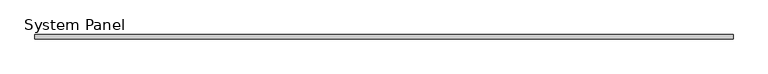
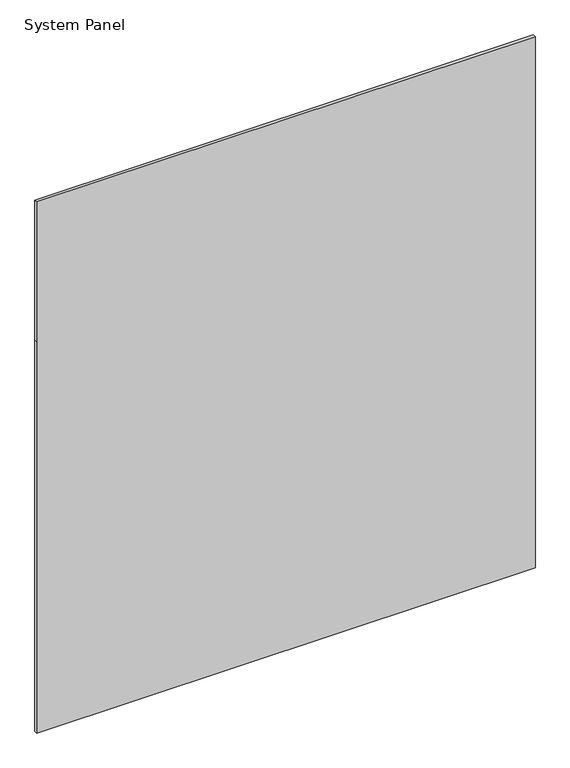
"""IFC4 building model written with IfcOpenShell, lengths in millimetres: plate geometry, System Panel : 로이복층유리_16."""

import ifcopenshell
import ifcopenshell.guid

model = None  # the IFC model being written
_history = None  # IfcOwnerHistory: only IFC2X3 demands one
_inside = {}  # id of a spatial element -> (the spatial element, [elements in it])
_under = {}  # id of a project, library or spatial element -> (it, [spatial elements below it])
_declared = {}  # id of a project -> (the project, [libraries it declares])
_typed = {}  # id of a type object -> (the type object, [elements of that type])
_made_of = {}  # id of a material, layer set ... -> (it, [elements and type objects made of it])


def new_model(schema):
    """Start an empty IFC model of exactly this schema.

    Asked for "IFC4X3", IfcOpenShell would pick the latest addendum, in which some entities
    have other attributes; the version numbers below select the first issue.
    IFC2X3 requires an IfcOwnerHistory on every rooted entity: one is made here for all.
    """
    global model, _history
    if schema == "IFC4X3":
        model = ifcopenshell.file(schema_version=(4, 3, 0, 0))
    else:
        model = ifcopenshell.file(schema=schema)
    _inside.clear()
    _under.clear()
    _declared.clear()
    _typed.clear()
    _made_of.clear()
    _history = None
    if model.schema == "IFC2X3":
        org = make("IfcOrganization", Name="unknown")
        user = make(
            "IfcPersonAndOrganization",
            ThePerson=make("IfcPerson", FamilyName="unknown"),
            TheOrganization=org,
        )
        app = make(
            "IfcApplication",
            ApplicationDeveloper=org,
            Version="unknown",
            ApplicationFullName="unknown",
            ApplicationIdentifier="unknown",
        )
        _history = make(
            "IfcOwnerHistory",
            OwningUser=user,
            OwningApplication=app,
            ChangeAction="ADDED",
            CreationDate=0,
        )
    return model


def make(cls, **values):
    """One entity of the class cls with the attributes given. An attribute that is None is left unset."""
    return model.create_entity(
        cls, **{name: value for name, value in values.items() if value is not None}
    )


def rooted(cls, **values):
    """An entity with a GlobalId (a new one), such as an element, a storey or a relation."""
    return make(cls, GlobalId=ifcopenshell.guid.new(), OwnerHistory=_history, **values)


def si_unit(unit_type, name, prefix=None):
    """IfcSIUnit, for example si_unit("LENGTHUNIT", "METRE", prefix="MILLI")."""
    return make("IfcSIUnit", UnitType=unit_type, Prefix=prefix, Name=name)


def assignment(units):
    """IfcUnitAssignment: the units of a project."""
    return None if units is None else make("IfcUnitAssignment", Units=units)


def point(xyz):
    """IfcCartesianPoint."""
    return None if xyz is None else make("IfcCartesianPoint", Coordinates=xyz)


def direction(xyz):
    """IfcDirection."""
    return None if xyz is None else make("IfcDirection", DirectionRatios=xyz)


def frame(location, z_axis=None, x_axis=None):
    """IfcAxis2Placement3D, a coordinate frame: its origin and axes. An axis left out is left unset."""
    return make(
        "IfcAxis2Placement3D",
        Location=point(location),
        Axis=direction(z_axis),
        RefDirection=direction(x_axis),
    )


def origin():
    """The frame at (0, 0, 0) with its axes left unset."""
    return frame((0.0, 0.0, 0.0))


def place(relative_to, where):
    """IfcLocalPlacement: puts the frame where relative to a parent placement (None: the world)."""
    return make(
        "IfcLocalPlacement", PlacementRelTo=relative_to, RelativePlacement=where
    )


def context(
    kind, dimensions, precision=None, world=None, true_north=None, identifier=None
):
    """IfcGeometricRepresentationContext, for example the 3D "Model" context."""
    return make(
        "IfcGeometricRepresentationContext",
        ContextIdentifier=identifier,
        ContextType=kind,
        CoordinateSpaceDimension=dimensions,
        Precision=precision,
        WorldCoordinateSystem=world,
        TrueNorth=true_north,
    )


def project(units=None, contexts=None):
    """IfcProject with its units and contexts."""
    return rooted(
        "IfcProject",
        Name="project",
        RepresentationContexts=contexts,
        UnitsInContext=assignment(units),
    )


def spatial(cls, under=None, at=None, **own):
    """A site, building, storey or space (cls), placed at a placement, below another one or the project."""
    s = rooted(cls, ObjectPlacement=at, **own)
    if under is not None:
        _under.setdefault(under.id(), (under, []))[1].append(s)
    return s


def polyline(points):
    """IfcPolyline through the points."""
    return make("IfcPolyline", Points=[point(p) for p in points])


def outline(outer, holes=None, kind="AREA"):
    """IfcArbitraryClosedProfileDef: a profile drawn as a closed curve; with holes, ...WithVoids."""
    if holes is None:
        return make("IfcArbitraryClosedProfileDef", ProfileType=kind, OuterCurve=outer)
    return make(
        "IfcArbitraryProfileDefWithVoids",
        ProfileType=kind,
        OuterCurve=outer,
        InnerCurves=holes,
    )


def extrude(swept, where, along, depth):
    """IfcExtrudedAreaSolid: the profile swept, set in the frame where, extruded along a direction by depth."""
    return make(
        "IfcExtrudedAreaSolid",
        SweptArea=swept,
        Position=where,
        ExtrudedDirection=direction(along),
        Depth=depth,
    )


def shape(context_of_items, identifier, shape_type, items):
    """IfcShapeRepresentation: the items that make up one representation, for example the "Body"."""
    return make(
        "IfcShapeRepresentation",
        ContextOfItems=context_of_items,
        RepresentationIdentifier=identifier,
        RepresentationType=shape_type,
        Items=items,
    )


def source(mapping_origin, context_of_items, identifier, shape_type, items):
    """IfcRepresentationMap: a shape defined once, which mapped items show again and again."""
    return make(
        "IfcRepresentationMap",
        MappingOrigin=mapping_origin,
        MappedRepresentation=shape(context_of_items, identifier, shape_type, items),
    )


def transform(
    local_origin,
    x_axis=None,
    y_axis=None,
    z_axis=None,
    scale=None,
    scale2=None,
    scale3=None,
    uniform=True,
):
    """IfcCartesianTransformationOperator3D, or its non-uniform kind. x_axis, y_axis, z_axis: its Axis1, 2, 3."""
    if uniform:
        return make(
            "IfcCartesianTransformationOperator3D",
            Axis1=direction(x_axis),
            Axis2=direction(y_axis),
            LocalOrigin=point(local_origin),
            Scale=scale,
            Axis3=direction(z_axis),
        )
    return make(
        "IfcCartesianTransformationOperator3DnonUniform",
        Axis1=direction(x_axis),
        Axis2=direction(y_axis),
        LocalOrigin=point(local_origin),
        Scale=scale,
        Axis3=direction(z_axis),
        Scale2=scale2,
        Scale3=scale3,
    )


def mapped(mapping_source, mapping_target):
    """IfcMappedItem: shows the shape of a source again, moved by a transform."""
    return make(
        "IfcMappedItem", MappingSource=mapping_source, MappingTarget=mapping_target
    )


def made_of(thing, what):
    """Note that an element or type object is made of a material, layer set ...; save() writes the relation."""
    if what is not None:
        _made_of.setdefault(what.id(), (what, []))[1].append(thing)
    return thing


def element(
    cls,
    number,
    at=None,
    inside=None,
    cuts=None,
    type_object=None,
    material=None,
    context=None,
    identifier="Body",
    shape_type=None,
    held_by="IfcProductDefinitionShape",
    body=None,
    shapes=None,
    **own,
):
    """One element of the class cls, such as IfcWall. Its Tag is "e" and its number.

    at: its placement. inside: the storey or other place that contains it. cuts: it is an
    opening in that element (IfcRelVoidsElement). A single representation is given by context,
    identifier, shape_type and body (its items); several are given by shapes. held_by: the class
    of the entity that holds the representations. save() writes the other relations.
    """
    e = rooted(cls, Tag="e%d" % number, ObjectPlacement=at, **own)
    if body is not None:
        shapes = [shape(context, identifier, shape_type, body)]
    if shapes is not None:
        e.Representation = make(held_by, Representations=shapes)
    if inside is not None:
        _inside.setdefault(inside.id(), (inside, []))[1].append(e)
    if cuts is not None:
        rooted(
            "IfcRelVoidsElement", RelatingBuildingElement=cuts, RelatedOpeningElement=e
        )
    if type_object is not None:
        _typed.setdefault(type_object.id(), (type_object, []))[1].append(e)
    return made_of(e, material)


def aggregate(whole, parts):
    """IfcRelAggregates: a whole, such as a stair, and the parts it consists of."""
    return rooted("IfcRelAggregates", RelatingObject=whole, RelatedObjects=parts)


def save(model, path):
    """Write the relations noted so far, then the file.

    IfcRelAggregates (storeys below a building ...), IfcRelContainedInSpatialStructure (elements
    in a storey), IfcRelDefinesByType, IfcRelAssociatesMaterial and IfcRelDeclares: one each for
    every whole, place, type object, material and project.
    """
    for whole, parts in _under.values():
        aggregate(whole, parts)
    for where, things in _inside.values():
        rooted(
            "IfcRelContainedInSpatialStructure",
            RelatedElements=things,
            RelatingStructure=where,
        )
    for kind, things in _typed.values():
        rooted("IfcRelDefinesByType", RelatedObjects=things, RelatingType=kind)
    for what, things in _made_of.values():
        rooted("IfcRelAssociatesMaterial", RelatedObjects=things, RelatingMaterial=what)
    for by, libraries in _declared.values():
        rooted("IfcRelDeclares", RelatingContext=by, RelatedDefinitions=libraries)
    model.write(path)


def system_panel_2a2c7901(model_context):
    return source(origin(), model_context, "Body", "SweptSolid", [
        extrude(outline(polyline([(0.0, -1312.5), (0.0, 1312.5), (2177.5, 1312.5), (2955.0, 1312.5), (2955.0, -1312.5), (2177.5, -1312.5), (0.0, -1312.5)])), frame((0.0, -8.0, 0.0), z_axis=(0.0, 1.0, 0.0), x_axis=(0.0, 0.0, 1.0)), (0.0, 0.0, 1.0), 16.0),
    ])


if __name__ == "__main__":
    model = new_model("IFC4")
    model_context = context("Model", 3, world=origin())
    ifc_project = project(units=[si_unit("LENGTHUNIT", "METRE", prefix="MILLI")], contexts=[model_context])
    site = spatial("IfcSite", under=ifc_project)
    building = spatial("IfcBuilding", under=site)
    placement = place(None, origin())
    system_panel_shape = system_panel_2a2c7901(model_context)
    element("IfcPlate", 1, ObjectType="System Panel : 로이복층유리_16", at=placement, inside=building, context=model_context, shape_type="MappedRepresentation", body=[
        mapped(system_panel_shape, transform((0.0, 0.0, 0.0), x_axis=(1.0, 0.0, 0.0), y_axis=(0.0, 1.0, 0.0), z_axis=(0.0, 0.0, 1.0))),
    ])
    save(model, "model.ifc")

# Revit data of these elements
# Element 1 (IfcPlate, "System Panel : 로이복층유리_16")
#   Materials on its faces: "00_Glass_Glass"
# Materials
#   "00_Glass_Glass": class "Glass", colour RGB 218 227 224, transparency 0.85, Description = "Glass", Cost = 0, Image = none
